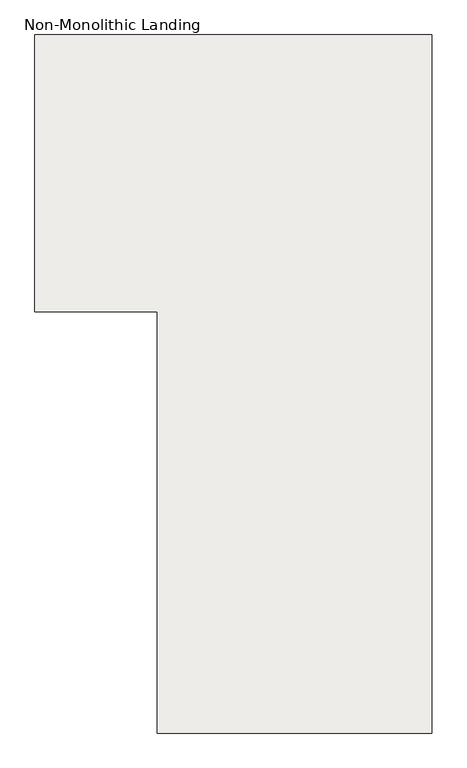
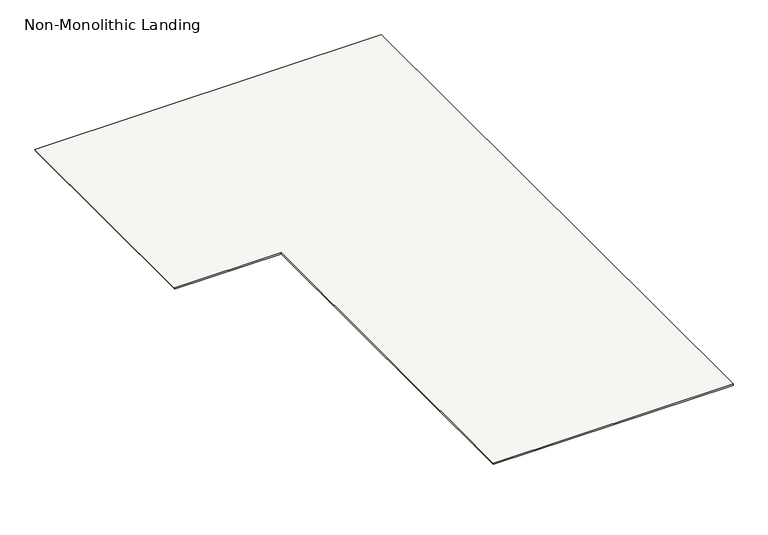
"""IFC4 building model written with IfcOpenShell, lengths in millimetres: slab geometry, Non-Monolithic Landing."""

import ifcopenshell
import ifcopenshell.guid

model = None  # the IFC model being written
_history = None  # IfcOwnerHistory: only IFC2X3 demands one
_inside = {}  # id of a spatial element -> (the spatial element, [elements in it])
_under = {}  # id of a project, library or spatial element -> (it, [spatial elements below it])
_declared = {}  # id of a project -> (the project, [libraries it declares])
_typed = {}  # id of a type object -> (the type object, [elements of that type])
_made_of = {}  # id of a material, layer set ... -> (it, [elements and type objects made of it])


def new_model(schema):
    """Start an empty IFC model of exactly this schema.

    Asked for "IFC4X3", IfcOpenShell would pick the latest addendum, in which some entities
    have other attributes; the version numbers below select the first issue.
    IFC2X3 requires an IfcOwnerHistory on every rooted entity: one is made here for all.
    """
    global model, _history
    if schema == "IFC4X3":
        model = ifcopenshell.file(schema_version=(4, 3, 0, 0))
    else:
        model = ifcopenshell.file(schema=schema)
    _inside.clear()
    _under.clear()
    _declared.clear()
    _typed.clear()
    _made_of.clear()
    _history = None
    if model.schema == "IFC2X3":
        org = make("IfcOrganization", Name="unknown")
        user = make(
            "IfcPersonAndOrganization",
            ThePerson=make("IfcPerson", FamilyName="unknown"),
            TheOrganization=org,
        )
        app = make(
            "IfcApplication",
            ApplicationDeveloper=org,
            Version="unknown",
            ApplicationFullName="unknown",
            ApplicationIdentifier="unknown",
        )
        _history = make(
            "IfcOwnerHistory",
            OwningUser=user,
            OwningApplication=app,
            ChangeAction="ADDED",
            CreationDate=0,
        )
    return model


def make(cls, **values):
    """One entity of the class cls with the attributes given. An attribute that is None is left unset."""
    return model.create_entity(
        cls, **{name: value for name, value in values.items() if value is not None}
    )


def rooted(cls, **values):
    """An entity with a GlobalId (a new one), such as an element, a storey or a relation."""
    return make(cls, GlobalId=ifcopenshell.guid.new(), OwnerHistory=_history, **values)


def si_unit(unit_type, name, prefix=None):
    """IfcSIUnit, for example si_unit("LENGTHUNIT", "METRE", prefix="MILLI")."""
    return make("IfcSIUnit", UnitType=unit_type, Prefix=prefix, Name=name)


def assignment(units):
    """IfcUnitAssignment: the units of a project."""
    return None if units is None else make("IfcUnitAssignment", Units=units)


def point(xyz):
    """IfcCartesianPoint."""
    return None if xyz is None else make("IfcCartesianPoint", Coordinates=xyz)


def direction(xyz):
    """IfcDirection."""
    return None if xyz is None else make("IfcDirection", DirectionRatios=xyz)


def frame(location, z_axis=None, x_axis=None):
    """IfcAxis2Placement3D, a coordinate frame: its origin and axes. An axis left out is left unset."""
    return make(
        "IfcAxis2Placement3D",
        Location=point(location),
        Axis=direction(z_axis),
        RefDirection=direction(x_axis),
    )


def origin():
    """The frame at (0, 0, 0) with its axes left unset."""
    return frame((0.0, 0.0, 0.0))


def place(relative_to, where):
    """IfcLocalPlacement: puts the frame where relative to a parent placement (None: the world)."""
    return make(
        "IfcLocalPlacement", PlacementRelTo=relative_to, RelativePlacement=where
    )


def context(
    kind, dimensions, precision=None, world=None, true_north=None, identifier=None
):
    """IfcGeometricRepresentationContext, for example the 3D "Model" context."""
    return make(
        "IfcGeometricRepresentationContext",
        ContextIdentifier=identifier,
        ContextType=kind,
        CoordinateSpaceDimension=dimensions,
        Precision=precision,
        WorldCoordinateSystem=world,
        TrueNorth=true_north,
    )


def project(units=None, contexts=None):
    """IfcProject with its units and contexts."""
    return rooted(
        "IfcProject",
        Name="project",
        RepresentationContexts=contexts,
        UnitsInContext=assignment(units),
    )


def spatial(cls, under=None, at=None, **own):
    """A site, building, storey or space (cls), placed at a placement, below another one or the project."""
    s = rooted(cls, ObjectPlacement=at, **own)
    if under is not None:
        _under.setdefault(under.id(), (under, []))[1].append(s)
    return s


def faces_of(points, faces, orient=None, outer=None):
    """IfcFace entities. A face is a list of loops; a loop is a list of indices into points, from 0.

    orient and outer hold one flag for each loop. By default every Orientation is true, the
    first loop of a face is its IfcFaceOuterBound and the others are IfcFaceBound.
    """
    made = []
    for i, loops in enumerate(faces):
        bounds = []
        for j, loop in enumerate(loops):
            is_outer = j == 0 if outer is None else outer[i][j]
            bounds.append(
                make(
                    "IfcFaceOuterBound" if is_outer else "IfcFaceBound",
                    Bound=make("IfcPolyLoop", Polygon=[points[k] for k in loop]),
                    Orientation=True if orient is None else orient[i][j],
                )
            )
        made.append(make("IfcFace", Bounds=bounds))
    return made


def faceted_brep(points, faces, orient=None, outer=None, voids=None):
    """IfcFacetedBrep: a solid bounded by flat faces; with voids (closed shells), ...WithVoids."""
    shared = [point(p) for p in points]
    hull = make("IfcClosedShell", CfsFaces=faces_of(shared, faces, orient, outer))
    if voids is None:
        return make("IfcFacetedBrep", Outer=hull)
    return make(
        "IfcFacetedBrepWithVoids",
        Outer=hull,
        Voids=[
            make(cls, CfsFaces=faces_of(shared, fs, o, b)) for cls, fs, o, b in voids
        ],
    )


def shape(context_of_items, identifier, shape_type, items):
    """IfcShapeRepresentation: the items that make up one representation, for example the "Body"."""
    return make(
        "IfcShapeRepresentation",
        ContextOfItems=context_of_items,
        RepresentationIdentifier=identifier,
        RepresentationType=shape_type,
        Items=items,
    )


def source(mapping_origin, context_of_items, identifier, shape_type, items):
    """IfcRepresentationMap: a shape defined once, which mapped items show again and again."""
    return make(
        "IfcRepresentationMap",
        MappingOrigin=mapping_origin,
        MappedRepresentation=shape(context_of_items, identifier, shape_type, items),
    )


def transform(
    local_origin,
    x_axis=None,
    y_axis=None,
    z_axis=None,
    scale=None,
    scale2=None,
    scale3=None,
    uniform=True,
):
    """IfcCartesianTransformationOperator3D, or its non-uniform kind. x_axis, y_axis, z_axis: its Axis1, 2, 3."""
    if uniform:
        return make(
            "IfcCartesianTransformationOperator3D",
            Axis1=direction(x_axis),
            Axis2=direction(y_axis),
            LocalOrigin=point(local_origin),
            Scale=scale,
            Axis3=direction(z_axis),
        )
    return make(
        "IfcCartesianTransformationOperator3DnonUniform",
        Axis1=direction(x_axis),
        Axis2=direction(y_axis),
        LocalOrigin=point(local_origin),
        Scale=scale,
        Axis3=direction(z_axis),
        Scale2=scale2,
        Scale3=scale3,
    )


def mapped(mapping_source, mapping_target):
    """IfcMappedItem: shows the shape of a source again, moved by a transform."""
    return make(
        "IfcMappedItem", MappingSource=mapping_source, MappingTarget=mapping_target
    )


def made_of(thing, what):
    """Note that an element or type object is made of a material, layer set ...; save() writes the relation."""
    if what is not None:
        _made_of.setdefault(what.id(), (what, []))[1].append(thing)
    return thing


def element(
    cls,
    number,
    at=None,
    inside=None,
    cuts=None,
    type_object=None,
    material=None,
    context=None,
    identifier="Body",
    shape_type=None,
    held_by="IfcProductDefinitionShape",
    body=None,
    shapes=None,
    **own,
):
    """One element of the class cls, such as IfcWall. Its Tag is "e" and its number.

    at: its placement. inside: the storey or other place that contains it. cuts: it is an
    opening in that element (IfcRelVoidsElement). A single representation is given by context,
    identifier, shape_type and body (its items); several are given by shapes. held_by: the class
    of the entity that holds the representations. save() writes the other relations.
    """
    e = rooted(cls, Tag="e%d" % number, ObjectPlacement=at, **own)
    if body is not None:
        shapes = [shape(context, identifier, shape_type, body)]
    if shapes is not None:
        e.Representation = make(held_by, Representations=shapes)
    if inside is not None:
        _inside.setdefault(inside.id(), (inside, []))[1].append(e)
    if cuts is not None:
        rooted(
            "IfcRelVoidsElement", RelatingBuildingElement=cuts, RelatedOpeningElement=e
        )
    if type_object is not None:
        _typed.setdefault(type_object.id(), (type_object, []))[1].append(e)
    return made_of(e, material)


def aggregate(whole, parts):
    """IfcRelAggregates: a whole, such as a stair, and the parts it consists of."""
    return rooted("IfcRelAggregates", RelatingObject=whole, RelatedObjects=parts)


def save(model, path):
    """Write the relations noted so far, then the file.

    IfcRelAggregates (storeys below a building ...), IfcRelContainedInSpatialStructure (elements
    in a storey), IfcRelDefinesByType, IfcRelAssociatesMaterial and IfcRelDeclares: one each for
    every whole, place, type object, material and project.
    """
    for whole, parts in _under.values():
        aggregate(whole, parts)
    for where, things in _inside.values():
        rooted(
            "IfcRelContainedInSpatialStructure",
            RelatedElements=things,
            RelatingStructure=where,
        )
    for kind, things in _typed.values():
        rooted("IfcRelDefinesByType", RelatedObjects=things, RelatingType=kind)
    for what, things in _made_of.values():
        rooted("IfcRelAssociatesMaterial", RelatedObjects=things, RelatingMaterial=what)
    for by, libraries in _declared.values():
        rooted("IfcRelDeclares", RelatingContext=by, RelatedDefinitions=libraries)
    model.write(path)


def non_monolithic_landing_1176e692(model_context):
    return source(origin(), model_context, "Body", "Brep", [
        faceted_brep([(-14150.0, 12030.4345331, 20000.0), (-13625.0, 12030.4345331, 20000.0), (-13625.0, 10220.4345331, 20000.0), (-12444.9411574, 10220.4345331, 20000.0), (-12444.9411574, 13220.4345331, 20000.0), (-14150.0, 13220.4345331, 20000.0), (-13625.0, 10220.4345331, 19994.0), (-13625.0, 12030.4345331, 19994.0), (-14149.15, 12030.4345331, 19994.0), (-14149.15, 13220.4345331, 19994.0), (-12444.9411574, 13220.4345331, 19994.0), (-12444.9411574, 10220.4345331, 19994.0)], [[[0, 1, 2, 3, 4, 5]], [[6, 7, 8, 9, 10, 11]], [[5, 4, 10, 9]], [[1, 0, 8, 7]], [[2, 1, 7, 6]], [[3, 2, 6, 11]], [[4, 3, 11, 10]], [[0, 5, 9, 8]]]),
    ])


if __name__ == "__main__":
    model = new_model("IFC4")
    model_context = context("Model", 3, world=origin())
    ifc_project = project(units=[si_unit("LENGTHUNIT", "METRE", prefix="MILLI")], contexts=[model_context])
    site = spatial("IfcSite", under=ifc_project)
    building = spatial("IfcBuilding", under=site)
    placement = place(None, origin())
    non_monolithic_landing_shape = non_monolithic_landing_1176e692(model_context)
    element("IfcSlab", 1, ObjectType="Non-Monolithic Landing", at=placement, inside=building, context=model_context, shape_type="MappedRepresentation", body=[
        mapped(non_monolithic_landing_shape, transform((0.0, 0.0, 0.0), x_axis=(1.0, 0.0, 0.0), y_axis=(0.0, 1.0, 0.0), z_axis=(0.0, 0.0, 1.0))),
    ])
    save(model, "model.ifc")

# Revit data of these elements
# Element 1 (IfcSlab, "Non-Monolithic Landing")
#   Materials on its faces: "Steel, Paint Finish, Dark Gray"
# Materials
#   "Steel, Paint Finish, Dark Gray": class "Metal", colour RGB 89 89 89, transparency 0, Description = "Steel, paint finish, dark gray, glossy", Cost = 0
